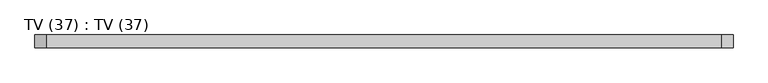
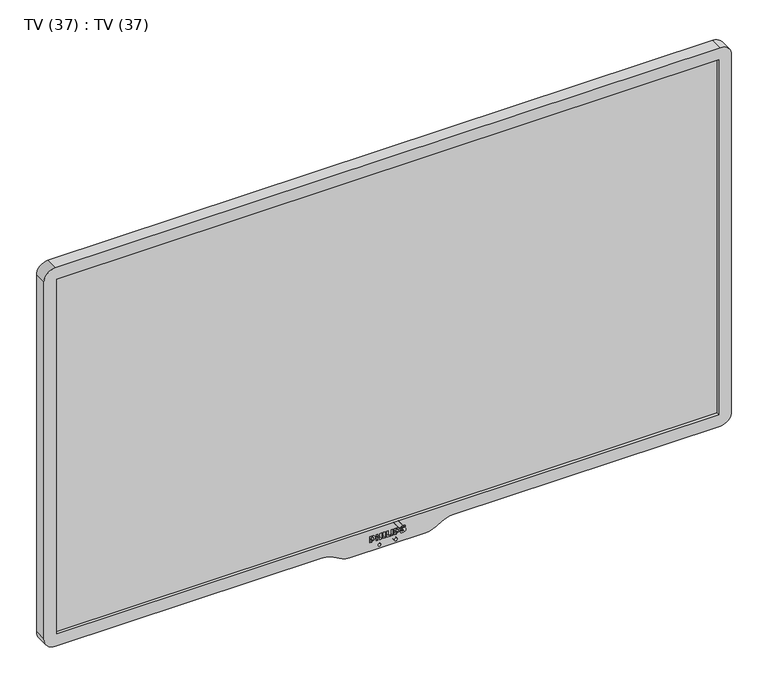
"""IFC4 building model written with IfcOpenShell, lengths in millimetres: furniture geometry, TV (37) : TV (37)."""

from ifc_helpers import new_model, si_unit, frame, origin, place, context, project, spatial, polyline, circle_curve, source, transform, mapped, element, save
from ifc_brep_helpers import plane_surface, cylinder_surface, revolved_surface, advanced_brep


def tv_37_tv_37_5d5eb749(model_context):
    return source(origin(), model_context, "Body", "AdvancedBrep", [
        advanced_brep(
        [(525.0, 20.0, 707.0), (543.0, 20.0, 689.0), (543.0, 20.0, 93.0), (525.0, 20.0, 75.0), (104.5344914, 20.0, 75.0), (85.2842297, 20.0, 69.9204298), (76.7494006, 20.0, 64.7092215), (60.0, 20.0, 60.0), (-60.0, 20.0, 60.0), (-76.7494006, 20.0, 64.7092215), (-85.2842297, 20.0, 69.9204298), (-104.5344914, 20.0, 75.0), (-525.0, 20.0, 75.0), (-543.0, 20.0, 93.0), (-543.0, 20.0, 689.0), (-525.0, 20.0, 707.0), (-28.3208351, 20.0, 73.6143863), (-25.3881417, 20.0, 73.6143863), (-25.3881417, 20.0, 75.713327), (-23.8490711, 20.0, 75.713327), (-23.8490711, 20.0, 83.6143863), (-28.3208351, 20.0, 83.6143863), (10.7374483, 20.0, 73.6143863), (13.6701416, 20.0, 73.6143863), (13.6701416, 20.0, 75.713327), (15.2092122, 20.0, 75.713327), (15.2092122, 20.0, 83.6143863), (10.7374483, 20.0, 83.6143863), (-18.3208351, 20.0, 73.6143863), (-15.2945136, 20.0, 73.6143863), (-15.2945136, 20.0, 77.6169143), (-12.294946, 20.0, 77.6169143), (-12.294946, 20.0, 73.6143863), (-9.2953784, 20.0, 73.6143863), (-9.2953784, 20.0, 83.6143863), (-12.294946, 20.0, 83.6143863), (-12.294946, 20.0, 79.5808385), (-15.2945136, 20.0, 79.5808385), (-15.2945136, 20.0, 83.6143863), (-18.3208351, 20.0, 83.6143863), (-6.8850115, 20.0, 73.6143863), (-3.8854439, 20.0, 73.6143863), (-3.8854439, 20.0, 83.6143863), (-6.8850115, 20.0, 83.6143863), (-1.6357682, 20.0, 73.6143863), (4.202676, 20.0, 73.6143863), (4.202676, 20.0, 76.1143863), (1.256672, 20.0, 76.1143863), (1.256672, 20.0, 83.6143863), (-1.6357682, 20.0, 83.6143863), (5.4346412, 20.0, 73.6143863), (8.4342089, 20.0, 73.6143863), (8.4342089, 20.0, 83.6143863), (5.4346412, 20.0, 83.6143863), (27.4493251, 20.0, 80.9835972), (27.4493251, 20.0, 83.6143863), (22.4493251, 20.0, 83.6143863), (22.0533828, 20.0, 77.9521479), (24.5942727, 20.0, 77.0772494), (24.5942727, 20.0, 75.4953718), (20.2638046, 20.0, 76.1143863), (20.394824, 20.0, 73.6143863), (26.5352021, 20.0, 73.6143863), (27.0267965, 20.0, 79.1844622), (23.7837853, 20.0, 80.3988963), (24.0290241, 20.0, 81.3430853), (11.0, 20.0, 65.0774036), (15.0, 20.0, 65.0774036), (-11.0, 20.0, 65.0774036), (-15.0, 20.0, 65.0774036), (525.0, 0.0, 707.0), (-525.0, 0.0, 707.0), (-543.0, 0.0, 689.0), (-543.0, 0.0, 93.0), (-525.0, 0.0, 75.0), (-104.5344914, 0.0, 75.0), (-85.2842297, 0.0, 69.9204298), (-76.7494006, 0.0, 64.7092215), (-60.0, 0.0, 60.0), (60.0, 0.0, 60.0), (76.7494006, 0.0, 64.7092215), (85.2842297, 0.0, 69.9204298), (104.5344914, 0.0, 75.0), (525.0, 0.0, 75.0), (543.0, 0.0, 93.0), (543.0, 0.0, 689.0), (-28.3208351, 0.0, 73.6143863), (-28.3208351, 0.0, 83.6143863), (-23.8490711, 0.0, 83.6143863), (-23.8490711, 0.0, 75.713327), (-25.3881417, 0.0, 75.713327), (-25.3881417, 0.0, 73.6143863), (10.7374483, 0.0, 73.6143863), (10.7374483, 0.0, 83.6143863), (15.2092122, 0.0, 83.6143863), (15.2092122, 0.0, 75.713327), (13.6701416, 0.0, 75.713327), (13.6701416, 0.0, 73.6143863), (-18.3208351, 0.0, 73.6143863), (-18.3208351, 0.0, 83.6143863), (-15.2945136, 0.0, 83.6143863), (-15.2945136, 0.0, 79.5808385), (-12.294946, 0.0, 79.5808385), (-12.294946, 0.0, 83.6143863), (-9.2953784, 0.0, 83.6143863), (-9.2953784, 0.0, 73.6143863), (-12.294946, 0.0, 73.6143863), (-12.294946, 0.0, 77.6169143), (-15.2945136, 0.0, 77.6169143), (-15.2945136, 0.0, 73.6143863), (-6.8850115, 0.0, 73.6143863), (-6.8850115, 0.0, 83.6143863), (-3.8854439, 0.0, 83.6143863), (-3.8854439, 0.0, 73.6143863), (-1.6357682, 0.0, 73.6143863), (-1.6357682, 0.0, 83.6143863), (1.256672, 0.0, 83.6143863), (1.256672, 0.0, 76.1143863), (4.202676, 0.0, 76.1143863), (4.202676, 0.0, 73.6143863), (5.4346412, 0.0, 73.6143863), (5.4346412, 0.0, 83.6143863), (8.4342089, 0.0, 83.6143863), (8.4342089, 0.0, 73.6143863), (27.4493251, 0.0, 80.9835972), (24.0290241, 0.0, 81.3430853), (23.7837853, 0.0, 80.3988963), (27.0267965, 0.0, 79.1844622), (26.5352021, 0.0, 73.6143863), (20.394824, 0.0, 73.6143863), (20.2638046, 0.0, 76.1143863), (24.5942727, 0.0, 75.4953718), (24.5942727, 0.0, 77.0772494), (22.0533828, 0.0, 77.9521479), (22.4493251, 0.0, 83.6143863), (27.4493251, 0.0, 83.6143863), (11.0, 0.0, 65.0774036), (15.0, 0.0, 65.0774036), (-11.0, 0.0, 65.0774036), (-15.0, 0.0, 65.0774036), (523.0, 0.0, 687.0), (523.0, 0.0, 95.0), (-523.0, 0.0, 95.0), (-523.0, 0.0, 687.0), (523.0, 5.0, 95.0), (523.0, 5.0, 687.0), (-523.0, 5.0, 687.0), (-523.0, 5.0, 95.0)],
        [
            (0, 1, circle_curve(frame((525.0, 20.0, 689.0), z_axis=(0.0, 1.0, 0.0), x_axis=(1.0, 0.0, 0.0)), 18.0)),
            (1, 2),
            (2, 3, circle_curve(frame((525.0, 20.0, 93.0), z_axis=(0.0, 1.0, 0.0), x_axis=(1.0, 0.0, 0.0)), 18.0)),
            (3, 4),
            (4, 5, circle_curve(frame((104.5344914, 20.0, 35.9834498), z_axis=(0.0, -1.0, 0.0), x_axis=(-1.0, 0.0, 0.0)), 39.0165502)),
            (5, 6),
            (6, 7, circle_curve(frame((60.0, 20.0, 92.1411073), z_axis=(0.0, 1.0, 0.0), x_axis=(-1.0, 0.0, 0.0)), 32.1411073)),
            (7, 8),
            (8, 9, circle_curve(frame((-60.0, 20.0, 92.1411073), z_axis=(0.0, 1.0, 0.0), x_axis=(1.0, 0.0, 0.0)), 32.1411073)),
            (9, 10),
            (10, 11, circle_curve(frame((-104.5344914, 20.0, 35.9834498), z_axis=(0.0, -1.0, 0.0), x_axis=(1.0, 0.0, 0.0)), 39.0165502)),
            (11, 12),
            (12, 13, circle_curve(frame((-525.0, 20.0, 93.0), z_axis=(0.0, 1.0, 0.0), x_axis=(1.0, 0.0, 0.0)), 18.0)),
            (13, 14),
            (14, 15, circle_curve(frame((-525.0, 20.0, 689.0), z_axis=(0.0, 1.0, 0.0), x_axis=(1.0, 0.0, 0.0)), 18.0)),
            (15, 0),
            (16, 17),
            (17, 18),
            (18, 19),
            (19, 20, circle_curve(frame((-23.8490711, 20.0, 79.6638566), z_axis=(0.0, -1.0, 0.0), x_axis=(1.0, 0.0, 0.0)), 3.9505297)),
            (20, 21),
            (21, 16),
            (22, 23),
            (23, 24),
            (24, 25),
            (25, 26, circle_curve(frame((15.2092122, 20.0, 79.6638566), z_axis=(0.0, -1.0, 0.0), x_axis=(1.0, 0.0, 0.0)), 3.9505297)),
            (26, 27),
            (27, 22),
            (28, 29),
            (29, 30),
            (30, 31),
            (31, 32),
            (32, 33),
            (33, 34),
            (34, 35),
            (35, 36),
            (36, 37),
            (37, 38),
            (38, 39),
            (39, 28),
            (40, 41),
            (41, 42),
            (42, 43),
            (43, 40),
            (44, 45),
            (45, 46),
            (46, 47),
            (47, 48),
            (48, 49),
            (49, 44),
            (50, 51),
            (51, 52),
            (52, 53),
            (53, 50),
            (54, 55),
            (55, 56, circle_curve(frame((24.9493251, 20.0, 75.1076941), z_axis=(0.0, -1.0, 0.0), x_axis=(1.0, 0.0, 0.0)), 8.866443)),
            (56, 57, circle_curve(frame((23.3029632, 20.0, 80.7097314), z_axis=(0.0, -1.0, 0.0), x_axis=(1.0, 0.0, 0.0)), 3.0274937)),
            (57, 58, circle_curve(frame((27.9711764, 20.0, 91.0115792), z_axis=(0.0, -1.0, 0.0), x_axis=(1.0, 0.0, 0.0)), 14.3376786)),
            (58, 59, circle_curve(frame((24.4025933, 20.0, 76.2863106), z_axis=(0.0, 1.0, 0.0), x_axis=(1.0, 0.0, 0.0)), 0.8138336)),
            (59, 60, circle_curve(frame((23.2045241, 20.0, 81.2299787), z_axis=(0.0, 1.0, 0.0), x_axis=(1.0, 0.0, 0.0)), 5.9006031)),
            (60, 61),
            (61, 62, circle_curve(frame((23.4650131, 20.0, 83.5176437), z_axis=(0.0, -1.0, 0.0), x_axis=(1.0, 0.0, 0.0)), 10.3682481)),
            (62, 63, circle_curve(frame((25.640587, 20.0, 76.5000729), z_axis=(0.0, -1.0, 0.0), x_axis=(1.0, 0.0, 0.0)), 3.0211791)),
            (63, 64, circle_curve(frame((20.0257494, 20.0, 65.4262115), z_axis=(0.0, -1.0, 0.0), x_axis=(1.0, 0.0, 0.0)), 15.4371022)),
            (64, 65, circle_curve(frame((24.0290241, 20.0, 80.8391423), z_axis=(0.0, 1.0, 0.0), x_axis=(1.0, 0.0, 0.0)), 0.503943)),
            (65, 54, circle_curve(frame((24.7031863, 20.0, 71.3065717), z_axis=(0.0, 1.0, 0.0), x_axis=(1.0, 0.0, 0.0)), 10.0591302)),
            (66, 67, circle_curve(frame((13.0, 20.0, 65.0774036), z_axis=(0.0, -1.0, 0.0), x_axis=(1.0, 0.0, 0.0)), 2.0)),
            (67, 66, circle_curve(frame((13.0, 20.0, 65.0774036), z_axis=(0.0, -1.0, 0.0), x_axis=(1.0, 0.0, 0.0)), 2.0)),
            (68, 69, circle_curve(frame((-13.0, 20.0, 65.0774036), z_axis=(0.0, -1.0, 0.0), x_axis=(-1.0, 0.0, 0.0)), 2.0)),
            (69, 68, circle_curve(frame((-13.0, 20.0, 65.0774036), z_axis=(0.0, -1.0, 0.0), x_axis=(-1.0, 0.0, 0.0)), 2.0)),
            (70, 71),
            (71, 72, circle_curve(frame((-525.0, 0.0, 689.0), z_axis=(0.0, -1.0, 0.0), x_axis=(1.0, 0.0, 0.0)), 18.0)),
            (72, 73),
            (73, 74, circle_curve(frame((-525.0, 0.0, 93.0), z_axis=(0.0, -1.0, 0.0), x_axis=(1.0, 0.0, 0.0)), 18.0)),
            (74, 75),
            (75, 76, circle_curve(frame((-104.5344914, 0.0, 35.9834498), z_axis=(0.0, 1.0, 0.0), x_axis=(1.0, 0.0, 0.0)), 39.0165502)),
            (76, 77),
            (77, 78, circle_curve(frame((-60.0, 0.0, 92.1411073), z_axis=(0.0, -1.0, 0.0), x_axis=(1.0, 0.0, 0.0)), 32.1411073)),
            (78, 79),
            (79, 80, circle_curve(frame((60.0, 0.0, 92.1411073), z_axis=(0.0, -1.0, 0.0), x_axis=(-1.0, 0.0, 0.0)), 32.1411073)),
            (80, 81),
            (81, 82, circle_curve(frame((104.5344914, 0.0, 35.9834498), z_axis=(0.0, 1.0, 0.0), x_axis=(-1.0, 0.0, 0.0)), 39.0165502)),
            (82, 83),
            (83, 84, circle_curve(frame((525.0, 0.0, 93.0), z_axis=(0.0, -1.0, 0.0), x_axis=(1.0, 0.0, 0.0)), 18.0)),
            (84, 85),
            (85, 70, circle_curve(frame((525.0, 0.0, 689.0), z_axis=(0.0, -1.0, 0.0), x_axis=(1.0, 0.0, 0.0)), 18.0)),
            (86, 87),
            (87, 88),
            (88, 89, circle_curve(frame((-23.8490711, 0.0, 79.6638566), z_axis=(0.0, 1.0, 0.0), x_axis=(1.0, 0.0, 0.0)), 3.9505297)),
            (89, 90),
            (90, 91),
            (91, 86),
            (92, 93),
            (93, 94),
            (94, 95, circle_curve(frame((15.2092122, 0.0, 79.6638566), z_axis=(0.0, 1.0, 0.0), x_axis=(1.0, 0.0, 0.0)), 3.9505297)),
            (95, 96),
            (96, 97),
            (97, 92),
            (98, 99),
            (99, 100),
            (100, 101),
            (101, 102),
            (102, 103),
            (103, 104),
            (104, 105),
            (105, 106),
            (106, 107),
            (107, 108),
            (108, 109),
            (109, 98),
            (110, 111),
            (111, 112),
            (112, 113),
            (113, 110),
            (114, 115),
            (115, 116),
            (116, 117),
            (117, 118),
            (118, 119),
            (119, 114),
            (120, 121),
            (121, 122),
            (122, 123),
            (123, 120),
            (124, 125, circle_curve(frame((24.7031863, 0.0, 71.3065717), z_axis=(0.0, -1.0, 0.0), x_axis=(1.0, 0.0, 0.0)), 10.0591302)),
            (125, 126, circle_curve(frame((24.0290241, 0.0, 80.8391423), z_axis=(0.0, -1.0, 0.0), x_axis=(1.0, 0.0, 0.0)), 0.503943)),
            (126, 127, circle_curve(frame((20.0257494, 0.0, 65.4262115), z_axis=(0.0, 1.0, 0.0), x_axis=(1.0, 0.0, 0.0)), 15.4371022)),
            (127, 128, circle_curve(frame((25.640587, 0.0, 76.5000729), z_axis=(0.0, 1.0, 0.0), x_axis=(1.0, 0.0, 0.0)), 3.0211791)),
            (128, 129, circle_curve(frame((23.4650131, 0.0, 83.5176437), z_axis=(0.0, 1.0, 0.0), x_axis=(1.0, 0.0, 0.0)), 10.3682481)),
            (129, 130),
            (130, 131, circle_curve(frame((23.2045241, 0.0, 81.2299787), z_axis=(0.0, -1.0, 0.0), x_axis=(1.0, 0.0, 0.0)), 5.9006031)),
            (131, 132, circle_curve(frame((24.4025933, 0.0, 76.2863106), z_axis=(0.0, -1.0, 0.0), x_axis=(1.0, 0.0, 0.0)), 0.8138336)),
            (132, 133, circle_curve(frame((27.9711764, 0.0, 91.0115792), z_axis=(0.0, 1.0, 0.0), x_axis=(1.0, 0.0, 0.0)), 14.3376786)),
            (133, 134, circle_curve(frame((23.3029632, 0.0, 80.7097314), z_axis=(0.0, 1.0, 0.0), x_axis=(1.0, 0.0, 0.0)), 3.0274937)),
            (134, 135, circle_curve(frame((24.9493251, 0.0, 75.1076941), z_axis=(0.0, 1.0, 0.0), x_axis=(1.0, 0.0, 0.0)), 8.866443)),
            (135, 124),
            (136, 137, circle_curve(frame((13.0, 0.0, 65.0774036), z_axis=(0.0, 1.0, 0.0), x_axis=(1.0, 0.0, 0.0)), 2.0)),
            (137, 136, circle_curve(frame((13.0, 0.0, 65.0774036), z_axis=(0.0, 1.0, 0.0), x_axis=(1.0, 0.0, 0.0)), 2.0)),
            (138, 139, circle_curve(frame((-13.0, 0.0, 65.0774036), z_axis=(0.0, 1.0, 0.0), x_axis=(-1.0, 0.0, 0.0)), 2.0)),
            (139, 138, circle_curve(frame((-13.0, 0.0, 65.0774036), z_axis=(0.0, 1.0, 0.0), x_axis=(-1.0, 0.0, 0.0)), 2.0)),
            (140, 141),
            (141, 142),
            (142, 143),
            (143, 140),
            (0, 70),
            (85, 1),
            (84, 2),
            (83, 3),
            (82, 4),
            (81, 5),
            (80, 6),
            (79, 7),
            (78, 8),
            (77, 9),
            (76, 10),
            (75, 11),
            (74, 12),
            (73, 13),
            (72, 14),
            (71, 15),
            (16, 86),
            (91, 17),
            (90, 18),
            (89, 19),
            (88, 20),
            (87, 21),
            (22, 92),
            (97, 23),
            (96, 24),
            (95, 25),
            (94, 26),
            (93, 27),
            (28, 98),
            (109, 29),
            (108, 30),
            (107, 31),
            (106, 32),
            (105, 33),
            (104, 34),
            (103, 35),
            (102, 36),
            (101, 37),
            (100, 38),
            (99, 39),
            (40, 110),
            (113, 41),
            (112, 42),
            (111, 43),
            (44, 114),
            (119, 45),
            (118, 46),
            (117, 47),
            (116, 48),
            (115, 49),
            (50, 120),
            (123, 51),
            (122, 52),
            (121, 53),
            (54, 124),
            (135, 55),
            (134, 56),
            (133, 57),
            (132, 58),
            (131, 59),
            (130, 60),
            (129, 61),
            (128, 62),
            (127, 63),
            (126, 64),
            (125, 65),
            (66, 136),
            (137, 67),
            (68, 138),
            (139, 69),
            (144, 145),
            (145, 146),
            (146, 147),
            (147, 144),
            (144, 141),
            (140, 145),
            (143, 146),
            (142, 147),
        ],
        [
            plane_surface(frame((543.0, 20.0, 689.0), z_axis=(0.0, 1.0, 0.0), x_axis=(0.0, 0.0, -1.0))),
            plane_surface(frame((543.0, 0.0, 689.0), z_axis=(0.0, -1.0, 0.0), x_axis=(0.0, 0.0, 1.0))),
            cylinder_surface(frame((525.0, 0.0, 689.0), z_axis=(0.0, 1.0, 0.0), x_axis=(1.0, 0.0, 0.0)), 18.0),
            plane_surface(frame((543.0, 20.0, 689.0), z_axis=(1.0, 0.0, 0.0), x_axis=(0.0, -1.0, 0.0))),
            cylinder_surface(frame((525.0, 0.0, 93.0), z_axis=(0.0, 1.0, 0.0), x_axis=(1.0, 0.0, 0.0)), 18.0),
            plane_surface(frame((525.0, 20.0, 75.0), z_axis=(0.0, 0.0, -1.0), x_axis=(0.0, -1.0, 0.0))),
            revolved_surface(polyline([(65.5179412, 0.0, 35.9834498), (65.5179412, 20.0, 35.9834498)]), (104.5344914, 0.0, 35.9834498), (0.0, -1.0, 0.0)),
            plane_surface(frame((85.2842297, 20.0, 69.9204298), z_axis=(0.5211208324377472, 0.0, -0.8534829101976147), x_axis=(0.0, -1.0, 0.0))),
            cylinder_surface(frame((60.0, 0.0, 92.1411073), z_axis=(0.0, 1.0, 0.0), x_axis=(-1.0, 0.0, 0.0)), 32.1411073),
            plane_surface(frame((60.0, 20.0, 60.0), z_axis=(0.0, 0.0, -1.0), x_axis=(0.0, -1.0, 0.0))),
            cylinder_surface(frame((-60.0, 0.0, 92.1411073), z_axis=(0.0, 1.0, 0.0), x_axis=(1.0, 0.0, 0.0)), 32.1411073),
            plane_surface(frame((-76.7494006, 20.0, 64.7092215), z_axis=(-0.5211208324377438, 0.0, -0.8534829101976167), x_axis=(0.0, -1.0, 0.0))),
            revolved_surface(polyline([(-65.5179412, 0.0, 35.9834498), (-65.5179412, 20.0, 35.9834498)]), (-104.5344914, 0.0, 35.9834498), (0.0, -1.0, 0.0)),
            plane_surface(frame((-104.5344914, 20.0, 75.0), z_axis=(0.0, 0.0, -1.0), x_axis=(0.0, -1.0, 0.0))),
            cylinder_surface(frame((-525.0, 0.0, 93.0), z_axis=(0.0, 1.0, 0.0), x_axis=(1.0, 0.0, 0.0)), 18.0),
            plane_surface(frame((-543.0, 20.0, 93.0), z_axis=(-1.0, 0.0, 0.0), x_axis=(0.0, -1.0, 0.0))),
            cylinder_surface(frame((-525.0, 0.0, 689.0), z_axis=(0.0, 1.0, 0.0), x_axis=(1.0, 0.0, 0.0)), 18.0),
            plane_surface(frame((-525.0, 20.0, 707.0), z_axis=(0.0, 0.0, 1.0), x_axis=(0.0, -1.0, 0.0))),
            plane_surface(frame((-28.3208351, 20.0, 73.6143863), z_axis=(0.0, 0.0, 1.0), x_axis=(0.0, -1.0, 0.0))),
            plane_surface(frame((-25.3881417, 20.0, 73.6143863), z_axis=(-1.0, 0.0, 0.0), x_axis=(0.0, -1.0, 0.0))),
            plane_surface(frame((-25.3881417, 20.0, 75.713327), z_axis=(0.0, 0.0, 1.0), x_axis=(0.0, -1.0, 0.0))),
            revolved_surface(polyline([(-19.8985414, 0.0, 79.6638566), (-19.8985414, 20.0, 79.6638566)]), (-23.8490711, -10.0, 79.6638566), (0.0, -1.0, 0.0)),
            plane_surface(frame((-23.8490711, 20.0, 83.6143863), z_axis=(0.0, 0.0, -1.0), x_axis=(0.0, -1.0, 0.0))),
            plane_surface(frame((-28.3208351, 20.0, 83.6143863), z_axis=(1.0, 0.0, 0.0), x_axis=(0.0, -1.0, 0.0))),
            plane_surface(frame((10.7374483, 20.0, 73.6143863), z_axis=(0.0, 0.0, 1.0), x_axis=(0.0, -1.0, 0.0))),
            plane_surface(frame((13.6701416, 20.0, 73.6143863), z_axis=(-1.0, 0.0, 0.0), x_axis=(0.0, -1.0, 0.0))),
            plane_surface(frame((13.6701416, 20.0, 75.713327), z_axis=(0.0, 0.0, 1.0), x_axis=(0.0, -1.0, 0.0))),
            revolved_surface(polyline([(19.1597419, 0.0, 79.6638566), (19.1597419, 20.0, 79.6638566)]), (15.2092122, -10.0, 79.6638566), (0.0, -1.0, 0.0)),
            plane_surface(frame((15.2092122, 20.0, 83.6143863), z_axis=(0.0, 0.0, -1.0), x_axis=(0.0, -1.0, 0.0))),
            plane_surface(frame((10.7374483, 20.0, 83.6143863), z_axis=(1.0, 0.0, 0.0), x_axis=(0.0, -1.0, 0.0))),
            plane_surface(frame((-18.3208351, 20.0, 73.6143863), z_axis=(0.0, 0.0, 1.0), x_axis=(0.0, -1.0, 0.0))),
            plane_surface(frame((-15.2945136, 20.0, 73.6143863), z_axis=(-1.0, 0.0, 0.0), x_axis=(0.0, -1.0, 0.0))),
            plane_surface(frame((-15.2945136, 20.0, 77.6169143), z_axis=(0.0, 0.0, 1.0), x_axis=(0.0, -1.0, 0.0))),
            plane_surface(frame((-12.294946, 20.0, 77.6169143), z_axis=(1.0, 0.0, 0.0), x_axis=(0.0, -1.0, 0.0))),
            plane_surface(frame((-12.294946, 20.0, 73.6143863), z_axis=(0.0, 0.0, 1.0), x_axis=(0.0, -1.0, 0.0))),
            plane_surface(frame((-9.2953784, 20.0, 73.6143863), z_axis=(-1.0, 0.0, 0.0), x_axis=(0.0, -1.0, 0.0))),
            plane_surface(frame((-9.2953784, 20.0, 83.6143863), z_axis=(0.0, 0.0, -1.0), x_axis=(0.0, -1.0, 0.0))),
            plane_surface(frame((-12.294946, 20.0, 83.6143863), z_axis=(1.0, 0.0, 0.0), x_axis=(0.0, -1.0, 0.0))),
            plane_surface(frame((-12.294946, 20.0, 79.5808385), z_axis=(0.0, 0.0, -1.0), x_axis=(0.0, -1.0, 0.0))),
            plane_surface(frame((-15.2945136, 20.0, 79.5808385), z_axis=(-1.0, 0.0, 0.0), x_axis=(0.0, -1.0, 0.0))),
            plane_surface(frame((-15.2945136, 20.0, 83.6143863), z_axis=(0.0, 0.0, -1.0), x_axis=(0.0, -1.0, 0.0))),
            plane_surface(frame((-18.3208351, 20.0, 83.6143863), z_axis=(1.0, 0.0, 0.0), x_axis=(0.0, -1.0, 0.0))),
            plane_surface(frame((-6.8850115, 20.0, 73.6143863), z_axis=(0.0, 0.0, 1.0), x_axis=(0.0, -1.0, 0.0))),
            plane_surface(frame((-3.8854439, 20.0, 73.6143863), z_axis=(-1.0, 0.0, 0.0), x_axis=(0.0, -1.0, 0.0))),
            plane_surface(frame((-3.8854439, 20.0, 83.6143863), z_axis=(0.0, 0.0, -1.0), x_axis=(0.0, -1.0, 0.0))),
            plane_surface(frame((-6.8850115, 20.0, 83.6143863), z_axis=(1.0, 0.0, 0.0), x_axis=(0.0, -1.0, 0.0))),
            plane_surface(frame((-1.6357682, 20.0, 73.6143863), z_axis=(0.0, 0.0, 1.0), x_axis=(0.0, -1.0, 0.0))),
            plane_surface(frame((4.202676, 20.0, 73.6143863), z_axis=(-1.0, 0.0, 0.0), x_axis=(0.0, -1.0, 0.0))),
            plane_surface(frame((4.202676, 20.0, 76.1143863), z_axis=(0.0, 0.0, -1.0), x_axis=(0.0, -1.0, 0.0))),
            plane_surface(frame((1.256672, 20.0, 76.1143863), z_axis=(-1.0, 0.0, 0.0), x_axis=(0.0, -1.0, 0.0))),
            plane_surface(frame((1.256672, 20.0, 83.6143863), z_axis=(0.0, 0.0, -1.0), x_axis=(0.0, -1.0, 0.0))),
            plane_surface(frame((-1.6357682, 20.0, 83.6143863), z_axis=(1.0, 0.0, 0.0), x_axis=(0.0, -1.0, 0.0))),
            plane_surface(frame((5.4346412, 20.0, 73.6143863), z_axis=(0.0, 0.0, 1.0), x_axis=(0.0, -1.0, 0.0))),
            plane_surface(frame((8.4342089, 20.0, 73.6143863), z_axis=(-1.0, 0.0, 0.0), x_axis=(0.0, -1.0, 0.0))),
            plane_surface(frame((8.4342089, 20.0, 83.6143863), z_axis=(0.0, 0.0, -1.0), x_axis=(0.0, -1.0, 0.0))),
            plane_surface(frame((5.4346412, 20.0, 83.6143863), z_axis=(1.0, 0.0, 0.0), x_axis=(0.0, -1.0, 0.0))),
            plane_surface(frame((27.4493251, 20.0, 80.9835972), z_axis=(-1.0, 0.0, 0.0), x_axis=(0.0, -1.0, 0.0))),
            revolved_surface(polyline([(33.8157681, 0.0, 75.1076941), (33.8157681, 20.0, 75.1076941)]), (24.9493251, -10.0, 75.1076941), (0.0, -1.0, 0.0)),
            revolved_surface(polyline([(26.3304569, 0.0, 80.7097314), (26.3304569, 20.0, 80.7097314)]), (23.3029632, -10.0, 80.7097314), (0.0, -1.0, 0.0)),
            revolved_surface(polyline([(42.308855, 0.0, 91.0115792), (42.308855, 20.0, 91.0115792)]), (27.9711764, -10.0, 91.0115792), (0.0, -1.0, 0.0)),
            cylinder_surface(frame((24.4025933, -10.0, 76.2863106), z_axis=(0.0, 1.0, 0.0), x_axis=(1.0, 0.0, 0.0)), 0.8138336),
            cylinder_surface(frame((23.2045241, -10.0, 81.2299787), z_axis=(0.0, 1.0, 0.0), x_axis=(1.0, 0.0, 0.0)), 5.9006031),
            plane_surface(frame((20.2638046, 20.0, 76.1143863), z_axis=(0.9986295347545738, 0.0, 0.052335956242946256), x_axis=(0.0, -1.0, 0.0))),
            revolved_surface(polyline([(33.8332612, 0.0, 83.5176437), (33.8332612, 20.0, 83.5176437)]), (23.4650131, -10.0, 83.5176437), (0.0, -1.0, 0.0)),
            revolved_surface(polyline([(28.6617661, 0.0, 76.5000729), (28.6617661, 20.0, 76.5000729)]), (25.640587, -10.0, 76.5000729), (0.0, -1.0, 0.0)),
            revolved_surface(polyline([(35.4628516, 0.0, 65.4262115), (35.4628516, 20.0, 65.4262115)]), (20.0257494, -10.0, 65.4262115), (0.0, -1.0, 0.0)),
            cylinder_surface(frame((24.0290241, -10.0, 80.8391423), z_axis=(0.0, 1.0, 0.0), x_axis=(1.0, 0.0, 0.0)), 0.503943),
            cylinder_surface(frame((24.7031863, -10.0, 71.3065717), z_axis=(0.0, 1.0, 0.0), x_axis=(1.0, 0.0, 0.0)), 10.0591302),
            revolved_surface(polyline([(15.0, 0.0, 65.0774036), (15.0, 20.0, 65.0774036)]), (13.0, -10.0, 65.0774036), (0.0, -1.0, 0.0)),
            revolved_surface(polyline([(-15.0, 0.0, 65.0774036), (-15.0, 20.0, 65.0774036)]), (-13.0, -10.0, 65.0774036), (0.0, -1.0, 0.0)),
            plane_surface(frame((523.0, 5.0, 97.1300387), z_axis=(0.0, -1.0, 0.0), x_axis=(0.0, 0.0, -1.0))),
            plane_surface(frame((523.0, 0.0, 95.0), z_axis=(-1.0, 0.0, 0.0), x_axis=(0.0, 1.0, 0.0))),
            plane_surface(frame((523.0, 0.0, 687.0), z_axis=(0.0, 0.0, -1.0), x_axis=(0.0, 1.0, 0.0))),
            plane_surface(frame((-523.0, 0.0, 687.0), z_axis=(1.0, 0.0, 0.0), x_axis=(0.0, 1.0, 0.0))),
            plane_surface(frame((-523.0, 0.0, 95.0), z_axis=(0.0, 0.0, 1.0), x_axis=(0.0, 1.0, 0.0))),
        ],
        [
            (0, [[1, 2, 3, 4, 5, 6, 7, 8, 9, 10, 11, 12, 13, 14, 15, 16], [17, 18, 19, 20, 21, 22], [23, 24, 25, 26, 27, 28], [29, 30, 31, 32, 33, 34, 35, 36, 37, 38, 39, 40], [41, 42, 43, 44], [45, 46, 47, 48, 49, 50], [51, 52, 53, 54], [55, 56, 57, 58, 59, 60, 61, 62, 63, 64, 65, 66], [67, 68], [69, 70]]),
            (1, [[71, 72, 73, 74, 75, 76, 77, 78, 79, 80, 81, 82, 83, 84, 85, 86], [87, 88, 89, 90, 91, 92], [93, 94, 95, 96, 97, 98], [99, 100, 101, 102, 103, 104, 105, 106, 107, 108, 109, 110], [111, 112, 113, 114], [115, 116, 117, 118, 119, 120], [121, 122, 123, 124], [125, 126, 127, 128, 129, 130, 131, 132, 133, 134, 135, 136], [137, 138], [139, 140], [141, 142, 143, 144]]),
            (2, [[-1, 145, -86, 146]]),
            (3, [[-2, -146, -85, 147]]),
            (4, [[-3, -147, -84, 148]]),
            (5, [[-4, -148, -83, 149]]),
            (6, [[-5, -149, -82, 150]]),
            (7, [[-6, -150, -81, 151]]),
            (8, [[-7, -151, -80, 152]]),
            (9, [[-8, -152, -79, 153]]),
            (10, [[-9, -153, -78, 154]]),
            (11, [[-10, -154, -77, 155]]),
            (12, [[-11, -155, -76, 156]]),
            (13, [[-12, -156, -75, 157]]),
            (14, [[-13, -157, -74, 158]]),
            (15, [[-14, -158, -73, 159]]),
            (16, [[-15, -159, -72, 160]]),
            (17, [[-16, -160, -71, -145]]),
            (18, [[-17, 161, -92, 162]]),
            (19, [[-18, -162, -91, 163]]),
            (20, [[-19, -163, -90, 164]]),
            (21, [[-20, -164, -89, 165]]),
            (22, [[-21, -165, -88, 166]]),
            (23, [[-22, -166, -87, -161]]),
            (24, [[-23, 167, -98, 168]]),
            (25, [[-24, -168, -97, 169]]),
            (26, [[-25, -169, -96, 170]]),
            (27, [[-26, -170, -95, 171]]),
            (28, [[-27, -171, -94, 172]]),
            (29, [[-28, -172, -93, -167]]),
            (30, [[-29, 173, -110, 174]]),
            (31, [[-30, -174, -109, 175]]),
            (32, [[-31, -175, -108, 176]]),
            (33, [[-32, -176, -107, 177]]),
            (34, [[-33, -177, -106, 178]]),
            (35, [[-34, -178, -105, 179]]),
            (36, [[-35, -179, -104, 180]]),
            (37, [[-36, -180, -103, 181]]),
            (38, [[-37, -181, -102, 182]]),
            (39, [[-38, -182, -101, 183]]),
            (40, [[-39, -183, -100, 184]]),
            (41, [[-40, -184, -99, -173]]),
            (42, [[-41, 185, -114, 186]]),
            (43, [[-42, -186, -113, 187]]),
            (44, [[-43, -187, -112, 188]]),
            (45, [[-44, -188, -111, -185]]),
            (46, [[-45, 189, -120, 190]]),
            (47, [[-46, -190, -119, 191]]),
            (48, [[-47, -191, -118, 192]]),
            (49, [[-48, -192, -117, 193]]),
            (50, [[-49, -193, -116, 194]]),
            (51, [[-50, -194, -115, -189]]),
            (52, [[-51, 195, -124, 196]]),
            (53, [[-52, -196, -123, 197]]),
            (54, [[-53, -197, -122, 198]]),
            (55, [[-54, -198, -121, -195]]),
            (56, [[-55, 199, -136, 200]]),
            (57, [[-56, -200, -135, 201]]),
            (58, [[-57, -201, -134, 202]]),
            (59, [[-58, -202, -133, 203]]),
            (60, [[-59, -203, -132, 204]]),
            (61, [[-60, -204, -131, 205]]),
            (62, [[-61, -205, -130, 206]]),
            (63, [[-62, -206, -129, 207]]),
            (64, [[-63, -207, -128, 208]]),
            (65, [[-64, -208, -127, 209]]),
            (66, [[-65, -209, -126, 210]]),
            (67, [[-66, -210, -125, -199]]),
            (68, [[-67, 211, -138, 212]]),
            (68, [[-68, -212, -137, -211]]),
            (69, [[-69, 213, -140, 214]]),
            (69, [[-70, -214, -139, -213]]),
            (70, [[215, 216, 217, 218]]),
            (71, [[-215, 219, -141, 220]]),
            (72, [[-216, -220, -144, 221]]),
            (73, [[-217, -221, -143, 222]]),
            (74, [[-218, -222, -142, -219]]),
        ],
    ),
        advanced_brep(
        [(-25.1021039, 20.0, 81.3430853), (-24.316066, 20.0, 81.3430853), (-24.316066, 20.0, 77.6169143), (-25.1021039, 20.0, 77.6169143), (-25.1021039, 0.0, 81.3430853), (-25.1021039, 0.0, 77.6169143), (-24.316066, 0.0, 77.6169143), (-24.316066, 0.0, 81.3430853)],
        [
            (0, 1),
            (1, 2, circle_curve(frame((-24.316066, 20.0, 79.4799998), z_axis=(0.0, 1.0, 0.0), x_axis=(1.0, 0.0, 0.0)), 1.8630855)),
            (2, 3),
            (3, 0),
            (4, 5),
            (5, 6),
            (6, 7, circle_curve(frame((-24.316066, 0.0, 79.4799998), z_axis=(0.0, -1.0, 0.0), x_axis=(1.0, 0.0, 0.0)), 1.8630855)),
            (7, 4),
            (0, 4),
            (7, 1),
            (6, 2),
            (5, 3),
        ],
        [
            plane_surface(frame((543.0, 20.0, 689.0), z_axis=(0.0, 1.0, 0.0), x_axis=(0.0, 0.0, -1.0))),
            plane_surface(frame((543.0, 0.0, 689.0), z_axis=(0.0, -1.0, 0.0), x_axis=(0.0, 0.0, 1.0))),
            plane_surface(frame((-25.1021039, 20.0, 81.3430853), z_axis=(0.0, 0.0, 1.0), x_axis=(0.0, -1.0, 0.0))),
            cylinder_surface(frame((-24.316066, -10.0, 79.4799998), z_axis=(0.0, 1.0, 0.0), x_axis=(1.0, 0.0, 0.0)), 1.8630855),
            plane_surface(frame((-24.316066, 20.0, 77.6169143), z_axis=(0.0, 0.0, -1.0), x_axis=(0.0, -1.0, 0.0))),
            plane_surface(frame((-25.1021039, 20.0, 77.6169143), z_axis=(-1.0, 0.0, 0.0), x_axis=(0.0, -1.0, 0.0))),
        ],
        [
            (0, [[1, 2, 3, 4]]),
            (1, [[5, 6, 7, 8]]),
            (2, [[-1, 9, -8, 10]]),
            (3, [[-2, -10, -7, 11]]),
            (4, [[-3, -11, -6, 12]]),
            (5, [[-4, -12, -5, -9]]),
        ],
    ),
        advanced_brep(
        [(13.9561795, 20.0, 81.3430853), (14.7422174, 20.0, 81.3430853), (14.7422174, 20.0, 77.6169143), (13.9561795, 20.0, 77.6169143), (13.9561795, 0.0, 81.3430853), (13.9561795, 0.0, 77.6169143), (14.7422174, 0.0, 77.6169143), (14.7422174, 0.0, 81.3430853)],
        [
            (0, 1),
            (1, 2, circle_curve(frame((14.7422174, 20.0, 79.4799998), z_axis=(0.0, 1.0, 0.0), x_axis=(1.0, 0.0, 0.0)), 1.8630855)),
            (2, 3),
            (3, 0),
            (4, 5),
            (5, 6),
            (6, 7, circle_curve(frame((14.7422174, 0.0, 79.4799998), z_axis=(0.0, -1.0, 0.0), x_axis=(1.0, 0.0, 0.0)), 1.8630855)),
            (7, 4),
            (0, 4),
            (7, 1),
            (6, 2),
            (5, 3),
        ],
        [
            plane_surface(frame((543.0, 20.0, 689.0), z_axis=(0.0, 1.0, 0.0), x_axis=(0.0, 0.0, -1.0))),
            plane_surface(frame((543.0, 0.0, 689.0), z_axis=(0.0, -1.0, 0.0), x_axis=(0.0, 0.0, 1.0))),
            plane_surface(frame((13.9561795, 20.0, 81.3430853), z_axis=(0.0, 0.0, 1.0), x_axis=(0.0, -1.0, 0.0))),
            cylinder_surface(frame((14.7422174, -10.0, 79.4799998), z_axis=(0.0, 1.0, 0.0), x_axis=(1.0, 0.0, 0.0)), 1.8630855),
            plane_surface(frame((14.7422174, 20.0, 77.6169143), z_axis=(0.0, 0.0, -1.0), x_axis=(0.0, -1.0, 0.0))),
            plane_surface(frame((13.9561795, 20.0, 77.6169143), z_axis=(-1.0, 0.0, 0.0), x_axis=(0.0, -1.0, 0.0))),
        ],
        [
            (0, [[1, 2, 3, 4]]),
            (1, [[5, 6, 7, 8]]),
            (2, [[-1, 9, -8, 10]]),
            (3, [[-2, -10, -7, 11]]),
            (4, [[-3, -11, -6, 12]]),
            (5, [[-4, -12, -5, -9]]),
        ],
    ),
    ])


if __name__ == "__main__":
    model = new_model("IFC4")
    model_context = context("Model", 3, world=origin())
    ifc_project = project(units=[si_unit("LENGTHUNIT", "METRE", prefix="MILLI")], contexts=[model_context])
    site = spatial("IfcSite", under=ifc_project)
    building = spatial("IfcBuilding", under=site)
    placement = place(None, origin())
    tv_37_tv_37_shape = tv_37_tv_37_5d5eb749(model_context)
    element("IfcFurniture", 1, ObjectType="TV (37) : TV (37)", at=placement, inside=building, context=model_context, shape_type="MappedRepresentation", body=[
        mapped(tv_37_tv_37_shape, transform((0.0, 0.0, 0.0), x_axis=(1.0, 0.0, 0.0), y_axis=(0.0, 1.0, 0.0), z_axis=(0.0, 0.0, 1.0))),
    ])
    save(model, "model.ifc")

# Revit data of these elements
# Type "TV (37) : TV (37)"
#   Default Elevation = 0
# Element 1 (IfcFurniture, "TV (37) : TV (37)")
#   Materials on its faces: "_PHILIPS_Rahmen_Black_Hochglanz", "_PHILIPS_Rahmen_White_Hochglanz 2", "_PHILIPS_Rahmen_Silber", "_PHILIPS_Rahmen_Black_Matt", "_PHILIPS_Rahmen_Plexi", "_PHILIPS_Rahmen_Bildschirm"
# Materials
#   "_PHILIPS_Rahmen_Black_Hochglanz": class "Farbe", colour RGB 16 16 18, transparency 0
#   "_PHILIPS_Rahmen_White_Hochglanz 2": class "Farbe", colour RGB 255 255 255, transparency 0
#   "_PHILIPS_Rahmen_Silber": class "Farbe", colour RGB 139 145 150, transparency 0
#   "_PHILIPS_Rahmen_Black_Matt": class "Farbe", colour RGB 16 16 18, transparency 0
#   "_PHILIPS_Rahmen_Plexi": class "Glas", colour RGB 240 240 240, transparency 0.9
#   "_PHILIPS_Rahmen_Bildschirm": class "Farbe", colour RGB 33 33 39, transparency 0
